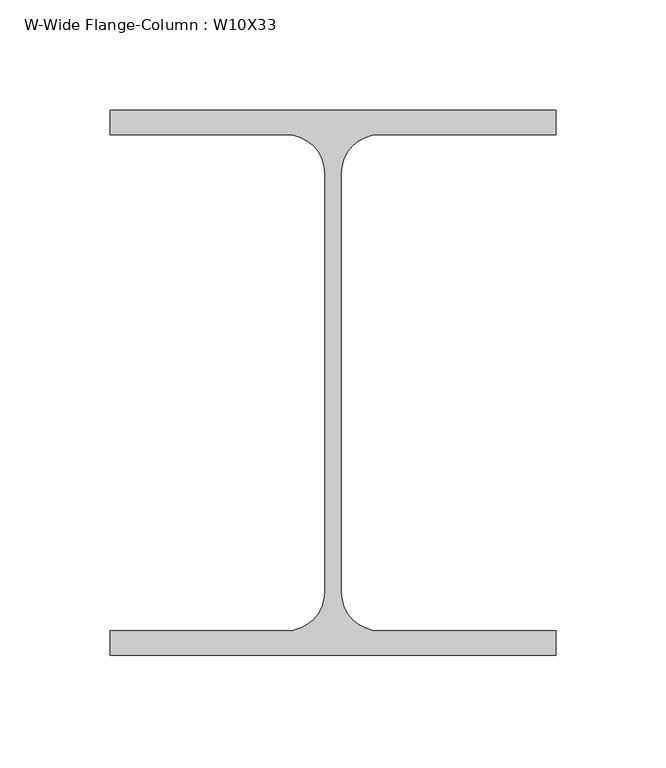
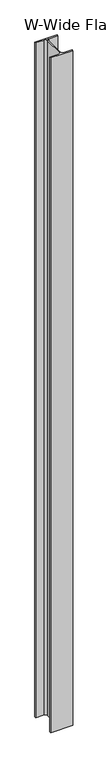
"""IFC4 building model written with IfcOpenShell, lengths in millimetres: column geometry, W-Wide Flange-Column : W10X33."""

from ifc_helpers import new_model, si_unit, point, frame, frame_2d, origin, place, context, project, spatial, polyline, circle_curve, trimmed, segment, composite_curve, outline, extrude, source, transform, mapped, element, save


def w_wide_flange_column_w10x33_69d6c3d7(model_context):
    return source(origin(), model_context, "Body", "SweptSolid", [
        extrude(outline(composite_curve([segment(polyline([(101.092, 123.571), (101.092, 112.522), (21.209, 112.522)]), True, "CONTINUOUS"), segment(trimmed(circle_curve(frame_2d((21.209, 94.996)), 17.526), [point((21.209, 112.522))], [point((3.683, 94.996))], True, "CARTESIAN"), True, "CONTINUOUS"), segment(polyline([(3.683, 94.996), (3.683, -94.996)]), True, "CONTINUOUS"), segment(trimmed(circle_curve(frame_2d((21.209, -94.996)), 17.526), [point((3.683, -94.996))], [point((21.209, -112.522))], True, "CARTESIAN"), True, "CONTINUOUS"), segment(polyline([(21.209, -112.522), (101.092, -112.522), (101.092, -123.571), (-101.092, -123.571), (-101.092, -112.522), (-21.209, -112.522)]), True, "CONTINUOUS"), segment(trimmed(circle_curve(frame_2d((-21.209, -94.996)), 17.526), [point((-21.209, -112.522))], [point((-3.683, -94.996))], True, "CARTESIAN"), True, "CONTINUOUS"), segment(polyline([(-3.683, -94.996), (-3.683, 94.996)]), True, "CONTINUOUS"), segment(trimmed(circle_curve(frame_2d((-21.209, 94.996)), 17.526), [point((-3.683, 94.996))], [point((-21.209, 112.522))], True, "CARTESIAN"), True, "CONTINUOUS"), segment(polyline([(-21.209, 112.522), (-101.092, 112.522), (-101.092, 123.571), (101.092, 123.571)]), True, "CONTINUOUS")], self_intersect=False)), frame((0.0, 0.0, 12566.65), z_axis=(0.0, 0.0, 1.0), x_axis=(1.0, 0.0, 0.0)), (0.0, 0.0, 1.0), 6483.35),
    ])


if __name__ == "__main__":
    model = new_model("IFC4")
    model_context = context("Model", 3, world=origin())
    ifc_project = project(units=[si_unit("LENGTHUNIT", "METRE", prefix="MILLI")], contexts=[model_context])
    site = spatial("IfcSite", under=ifc_project)
    building = spatial("IfcBuilding", under=site)
    placement = place(None, origin())
    w_wide_flange_column_w10x33_shape = w_wide_flange_column_w10x33_69d6c3d7(model_context)
    element("IfcColumn", 1, ObjectType="W-Wide Flange-Column : W10X33", at=placement, inside=building, context=model_context, shape_type="MappedRepresentation", body=[
        mapped(w_wide_flange_column_w10x33_shape, transform((0.0, 0.0, 0.0), x_axis=(1.0, 0.0, 0.0), y_axis=(0.0, 1.0, 0.0), z_axis=(0.0, 0.0, 1.0))),
    ])
    save(model, "model.ifc")

# Revit data of these elements
# Type "W-Wide Flange-Column : W10X33"
#   Assembly Code = "B10"
#   W = 33
#   bf = 0' - 7.96"
#   d = 0' - 9.73"
#   k = 0' - 1 1/8"
#   kr = 0' - 0.69"
#   tf = 0' - 0.435"
#   tw = 0' - 0.29"
#   A = 0.0674306 SF
#   Structural Material [instance default] = Steel ASTM A992
# Element 1 (IfcColumn, "W-Wide Flange-Column : W10X33")
#   Materials on its faces: "Steel ASTM A992"
# Materials
#   "Steel ASTM A992": class "Metal", colour RGB 199 199 199, transparency 0, Description = "Structural steel 50ksi", Cost = 0
